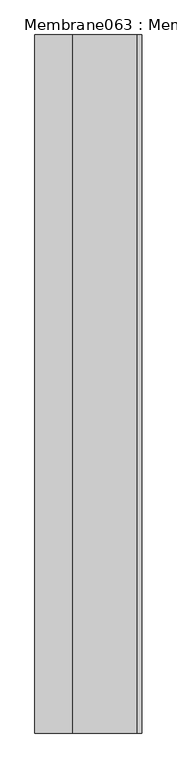
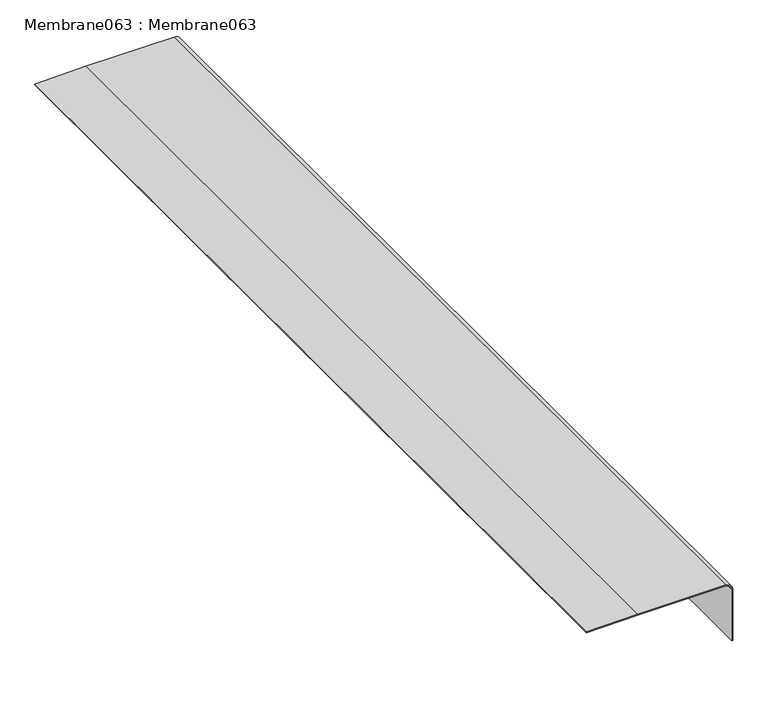
"""IFC4 building model written with IfcOpenShell, lengths in millimetres: proxy geometry, Membrane063 : Membrane063."""

from ifc_helpers import new_model, si_unit, point, frame, frame_2d, origin, place, context, project, spatial, polyline, circle_curve, trimmed, segment, composite_curve, outline, extrude, source, transform, mapped, element, save


def membrane063_membrane063_d60b8096(model_context):
    return source(origin(), model_context, "Body", "SweptSolid", [
        extrude(outline(composite_curve([segment(polyline([(40234.5370749, -4395.791679), (40120.9129128, -4395.791679), (40120.9129128, -4393.791679), (40234.5370749, -4393.791679)]), True, "CONTINUOUS"), segment(trimmed(circle_curve(frame_2d((40234.5370749, -4407.791679)), 14.0), [point((40234.5370749, -4393.791679))], [point((40248.5370749, -4407.791679))], False, "CARTESIAN"), True, "CONTINUOUS"), segment(polyline([(40248.5370749, -4407.791679), (40248.5370749, -4593.337414), (40247.0048323, -4699.8063764), (40245.0046252, -4699.8063764), (40246.5370749, -4593.3230233), (40246.5370749, -4407.791679)]), True, "CONTINUOUS"), segment(trimmed(circle_curve(frame_2d((40234.5370749, -4407.791679)), 12.0), [point((40246.5370749, -4407.791679))], [point((40234.5370749, -4395.791679))], True, "CARTESIAN"), True, "CONTINUOUS")], self_intersect=False)), frame((0.0, -1052.8906574, 0.0), z_axis=(0.0, 1.0, 0.0), x_axis=(0.0, 0.0, 1.0)), (0.0, 0.0, 1.0), 2000.0),
    ])


if __name__ == "__main__":
    model = new_model("IFC4")
    model_context = context("Model", 3, world=origin())
    ifc_project = project(units=[si_unit("LENGTHUNIT", "METRE", prefix="MILLI")], contexts=[model_context])
    site = spatial("IfcSite", under=ifc_project)
    building = spatial("IfcBuilding", under=site)
    placement = place(None, origin())
    membrane063_membrane063_shape = membrane063_membrane063_d60b8096(model_context)
    element("IfcBuildingElementProxy", 1, Name="Membrane063 : Membrane063", ObjectType="Membrane063 : Membrane063", at=placement, inside=building, context=model_context, shape_type="MappedRepresentation", body=[
        mapped(membrane063_membrane063_shape, transform((0.0, 0.0, 0.0), x_axis=(1.0, 0.0, 0.0), y_axis=(0.0, 1.0, 0.0), z_axis=(0.0, 0.0, 1.0))),
    ])
    save(model, "model.ifc")

# Revit data of these elements
# Type "Membrane063 : Membrane063"
#   NameOverride = "Membrane063"
# Element 1 (IfcBuildingElementProxy, "Membrane063 : Membrane063")
#   Materials on its faces: "THREE PLY BUILT UP ROOF MEMBRANE"
# Materials
#   "THREE PLY BUILT UP ROOF MEMBRANE": class "Unassigned", colour RGB 63 63 63, transparency 0
